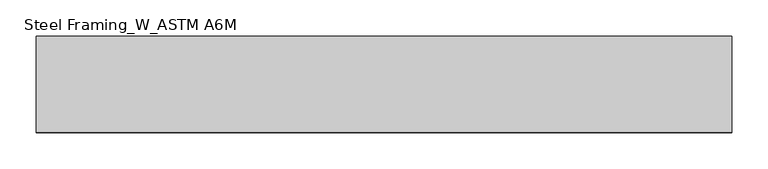
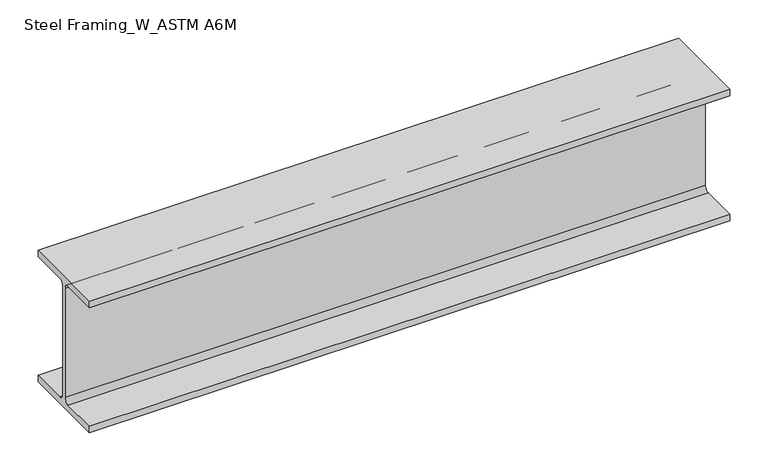
"""IFC4 building model written with IfcOpenShell, lengths in millimetres: beam geometry, Steel Framing_W_ASTM A6M : H_SB_AR_S02_W200x31.3_B6."""

from ifc_helpers import new_model, si_unit, point, frame, frame_2d, origin, place, context, project, spatial, polyline, circle_curve, trimmed, segment, composite_curve, outline, extrude, source, transform, mapped, element, save


def steel_framing_w_astm_a6m_5fdaaf4a(model_context):
    return source(origin(), model_context, "Body", "SweptSolid", [
        extrude(outline(composite_curve([segment(polyline([(67.0, -94.8), (67.0, -105.0), (-67.0, -105.0), (-67.0, -94.8), (-10.775, -94.8)]), True, "CONTINUOUS"), segment(trimmed(circle_curve(frame_2d((-10.775, -87.2)), 7.6), [point((-10.775, -94.8))], [point((-3.175, -87.2))], True, "CARTESIAN"), True, "CONTINUOUS"), segment(polyline([(-3.175, -87.2), (-3.175, 87.2)]), True, "CONTINUOUS"), segment(trimmed(circle_curve(frame_2d((-10.775, 87.2)), 7.6), [point((-3.175, 87.2))], [point((-10.775, 94.8))], True, "CARTESIAN"), True, "CONTINUOUS"), segment(polyline([(-10.775, 94.8), (-67.0, 94.8), (-67.0, 105.0), (67.0, 105.0), (67.0, 94.8), (10.775, 94.8)]), True, "CONTINUOUS"), segment(trimmed(circle_curve(frame_2d((10.775, 87.2)), 7.6), [point((10.775, 94.8))], [point((3.175, 87.2))], True, "CARTESIAN"), True, "CONTINUOUS"), segment(polyline([(3.175, 87.2), (3.175, -87.2)]), True, "CONTINUOUS"), segment(trimmed(circle_curve(frame_2d((10.775, -87.2)), 7.6), [point((3.175, -87.2))], [point((10.775, -94.8))], True, "CARTESIAN"), True, "CONTINUOUS"), segment(polyline([(10.775, -94.8), (67.0, -94.8)]), True, "CONTINUOUS")], self_intersect=False)), frame((-446.3, 0.0, 0.0), z_axis=(1.0, 0.0, 0.0), x_axis=(0.0, 1.0, 0.0)), (0.0, 0.0, 1.0), 966.6),
    ])


if __name__ == "__main__":
    model = new_model("IFC4")
    model_context = context("Model", 3, world=origin())
    ifc_project = project(units=[si_unit("LENGTHUNIT", "METRE", prefix="MILLI")], contexts=[model_context])
    site = spatial("IfcSite", under=ifc_project)
    building = spatial("IfcBuilding", under=site)
    placement = place(None, origin())
    steel_framing_w_astm_a6m_shape = steel_framing_w_astm_a6m_5fdaaf4a(model_context)
    element("IfcBeam", 1, ObjectType="Steel Framing_W_ASTM A6M : H_SB_AR_S02_W200x31.3_B6", at=placement, inside=building, context=model_context, shape_type="MappedRepresentation", body=[
        mapped(steel_framing_w_astm_a6m_shape, transform((0.0, 0.0, 0.0), x_axis=(1.0, 0.0, 0.0), y_axis=(0.0, 1.0, 0.0), z_axis=(0.0, 0.0, 1.0))),
    ])
    save(model, "model.ifc")

# Revit data of these elements
# Type "Steel Framing_W_ASTM A6M : H_SB_AR_S02_W200x31.3_B6"
#   Type Mark = "B6"
#   Section Name Key = "W8x21"
#   Width = 13.4 cm
#   Web Thickness = 0.635 cm
#   Web Fillet = 0.76 cm
#   Warping Constant = 40800.0 cm⁶
#   Torsional Moment of Inertia = 11.70 cm⁴
#   Section Area = 39.7 cm²
#   Plastic Modulus weak axis = 93.2 cm³
#   Plastic Modulus strong axis = 334.0 cm³
#   Perimeter = 0.93 m²/m
#   Nominal Weight = 31.30 kgf/m
#   Moment of Inertia weak axis = 407.00 cm⁴
#   Moment of Inertia strong axis = 3130.00 cm⁴
#   Height = 21.0 cm
#   Flange Thickness = 1.02 cm
#   Elastic Modulus weak axis = 60.8 cm³
#   Elastic Modulus strong axis = 298.0 cm³
#   Centroid Vertical = 10.5 cm
#   Centroid Horizontal = 6.7 cm
#   Length [instance default] = 1500 mm
#   Structural Material [instance default] = Steel, 45-345
#   Bolt Spacing = 0
#   Assembly Code = ""
# Element 1 (IfcBeam, "Steel Framing_W_ASTM A6M : H_SB_AR_S02_W200x31.3_B6")
#   Materials on its faces: "Steel, 45-345"
# Materials
#   "Steel, 45-345": class "Metal", colour RGB 189 187 185, transparency 0, Description = "Steel 345 MPa", Cost = 0
